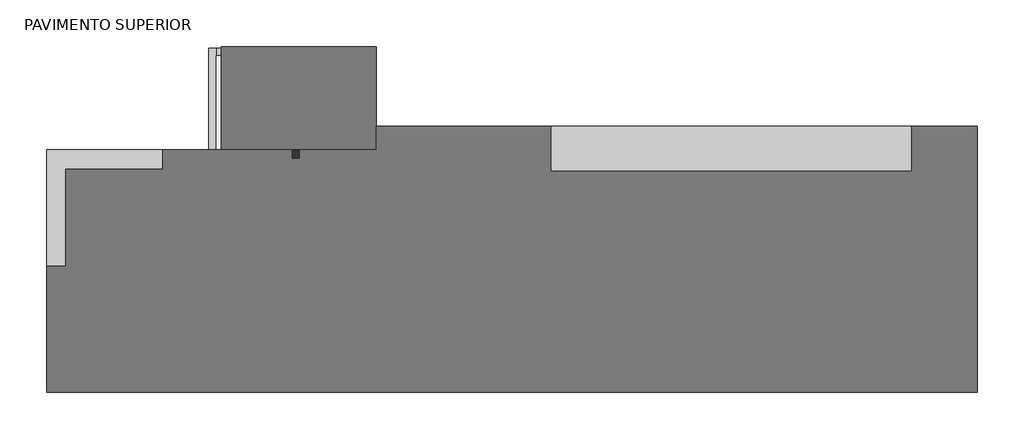
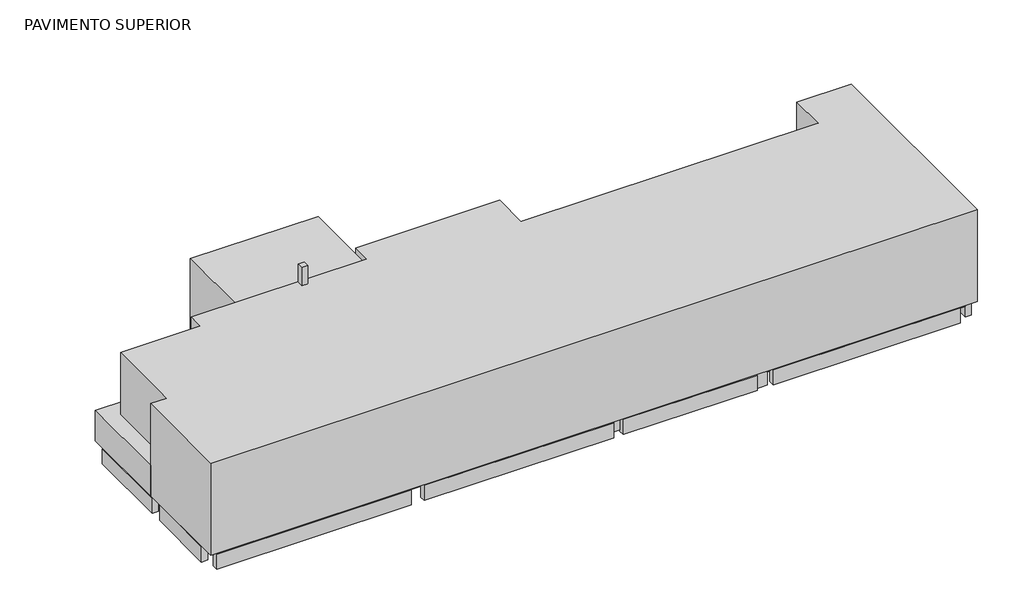
# One storey: 21 beams, 14 slabs, 2 proxies, 1 column.
"""IFC4 building model written with IfcOpenShell, lengths in millimetres."""

from ifc_helpers import new_model, si_unit, frame, origin, place, context, project, spatial, polyline, outline, extrude, faceted_brep, element, save

model = new_model("IFC4")

# Units and contexts
model_context = context("Model", 3, world=origin())
ifc_project = project(units=[si_unit("LENGTHUNIT", "METRE", prefix="MILLI")], contexts=[model_context])

# Site, building, storey
site = spatial("IfcSite", under=ifc_project)
building = spatial("IfcBuilding", under=site)
storey = spatial("IfcBuildingStorey", under=building, Name="PAVIMENTO SUPERIOR", Elevation=3600.0)

# Beams
placement = place(None, origin())
element("IfcBeam", 1, ObjectType="TQS - Viga retangular : 14.0 x 30.0", at=placement, inside=storey, context=model_context, shape_type="Brep", body=[
    faceted_brep([(10797.718693, -7454.5699847, 3530.0), (10797.718693, -7314.5699847, 3530.0), (9538.318693, -7314.5699847, 3530.0), (9538.318693, -7454.5699847, 3530.0), (10797.718693, -7454.5699847, 3230.0), (10797.718693, -7454.5699847, 3380.0), (9538.318693, -7454.5699847, 3380.0), (9538.318693, -7454.5699847, 3230.0), (10797.718693, -7314.5699847, 3230.0), (9538.318693, -7314.5699847, 3230.0), (10797.718693, -7314.5699847, 3380.0), (9538.318693, -7314.5699847, 3380.0)], [[[0, 1, 2, 3]], [[4, 5, 0, 3, 6, 7]], [[8, 4, 7, 9]], [[1, 10, 8, 9, 11, 2]], [[1, 0, 5, 4, 8, 10]], [[3, 2, 11, 9, 7, 6]]]),
])
element("IfcBeam", 2, ObjectType="TQS - Viga retangular : 14.0 x 50.0", at=placement, inside=storey, context=model_context, shape_type="Brep", body=[
    faceted_brep([(-5442.731307, -10953.5699847, 3530.0), (-5302.731307, -10953.5699847, 3530.0), (-5302.731307, -6553.3699847, 3530.0), (-5442.731307, -6553.3699847, 3530.0), (-5302.731307, -10953.5699847, 3380.0), (-5302.731307, -10953.5699847, 3030.0), (-5302.731307, -6553.3699847, 3030.0), (-5302.731307, -6553.3699847, 3380.0), (-5442.731307, -10953.5699847, 3030.0), (-5442.731307, -6553.3699847, 3030.0), (-5442.731307, -10953.5699847, 3380.0), (-5442.731307, -6553.3699847, 3380.0)], [[[0, 1, 2, 3]], [[1, 4, 5, 6, 7, 2]], [[5, 8, 9, 6]], [[8, 10, 0, 3, 11, 9]], [[1, 0, 10, 8, 5, 4]], [[3, 2, 7, 6, 9, 11]]]),
])
element("IfcBeam", 3, ObjectType="TQS - Viga retangular : 14.0 x 50.0", at=placement, inside=storey, context=model_context, shape_type="Brep", body=[
    faceted_brep([(-4442.481307, -4565.5699847, 3530.0), (-4442.481307, -4425.5699847, 3530.0), (-4512.281307, -4425.5699847, 3530.0), (-4702.281307, -4425.5699847, 3530.0), (-6440.281307, -4425.5699847, 3530.0), (-6440.281307, -4565.5699847, 3530.0), (-4702.281307, -4565.5699847, 3530.0), (-4512.281307, -4565.5699847, 3530.0), (-4442.481307, -4565.5699847, 3030.0), (-6440.281307, -4565.5699847, 3030.0), (-4702.281307, -4565.5699847, 3030.0), (-4512.281307, -4565.5699847, 3030.0), (-4442.481307, -4425.5699847, 3030.0), (-6440.281307, -4425.5699847, 3030.0), (-4702.281307, -4425.5699847, 3030.0), (-4512.281307, -4425.5699847, 3030.0), (-6440.281307, -4425.5699847, 3380.0)], [[[0, 1, 2, 3, 4, 5, 6, 7]], [[8, 0, 7, 6, 5, 9, 10, 11]], [[12, 8, 11, 10, 9, 13, 14, 15]], [[1, 12, 15, 14, 13, 16, 4, 3, 2]], [[1, 0, 8, 12]], [[5, 4, 16, 13, 9]]]),
])
element("IfcBeam", 4, ObjectType="TQS - Viga retangular : 14.0 x 50.0", at=placement, inside=storey, context=model_context, shape_type="Brep", body=[
    faceted_brep([(-4478.0679558, -6553.3699847, 3030.0), (-4478.0679558, -6413.3699847, 3030.0), (-4478.0679558, -6413.3699847, 3530.0), (-4478.0679558, -6450.0457433, 3530.0), (-4478.0679558, -6553.3699847, 3530.0), (-4478.0679558, -6553.3699847, 3380.0), (-6440.281307, -6413.3699847, 3530.0), (-6440.281307, -6553.3699847, 3530.0), (-5442.731307, -6553.3699847, 3530.0), (-5302.731307, -6553.3699847, 3530.0), (-4512.281307, -6413.3699847, 3530.0), (-4702.281307, -6413.3699847, 3530.0), (-6440.281307, -6553.3699847, 3030.0), (-5442.731307, -6553.3699847, 3030.0), (-5302.731307, -6553.3699847, 3030.0), (-6440.281307, -6413.3699847, 3030.0), (-4702.281307, -6413.3699847, 3030.0), (-4512.281307, -6413.3699847, 3030.0), (-6440.281307, -6413.3699847, 3380.0)], [[[0, 1, 2, 3, 4, 5]], [[6, 7, 8, 9, 4, 3, 2, 10, 11]], [[7, 12, 13, 14, 0, 5, 4, 9, 8]], [[1, 0, 14, 13, 12, 15, 16, 17]], [[2, 1, 17, 16, 15, 18, 6, 11, 10]], [[7, 6, 18, 15, 12]]]),
    faceted_brep([(-6840.281307, -6413.3699847, 3530.0), (-6840.281307, -6553.3699847, 3530.0), (-6840.281307, -6553.3699847, 3030.0), (-6840.281307, -6413.3699847, 3030.0), (-8589.281307, -6413.3699847, 3530.0), (-8589.281307, -6553.3699847, 3530.0), (-8589.281307, -6553.3699847, 3380.0), (-8589.281307, -6553.3699847, 3030.0), (-8589.281307, -6413.3699847, 3030.0), (-8589.281307, -6413.3699847, 3380.0)], [[[0, 1, 2, 3]], [[1, 0, 4, 5]], [[2, 1, 5, 6, 7]], [[3, 2, 7, 8]], [[0, 3, 8, 9, 4]], [[5, 4, 9, 8, 7, 6]]]),
    faceted_brep([(-8779.281307, -6413.3699847, 3530.0), (-8779.281307, -6553.3699847, 3530.0), (-8779.281307, -6553.3699847, 3380.0), (-8779.281307, -6553.3699847, 3030.0), (-8779.281307, -6413.3699847, 3030.0), (-8779.281307, -6413.3699847, 3380.0), (-12740.2813069, -6413.3699847, 3530.0), (-12740.2813069, -6553.3699847, 3530.0), (-12740.2813069, -6553.3699847, 3380.0), (-12740.2813069, -6553.3699847, 3030.0), (-12740.2813069, -6413.3699847, 3030.0), (-8780.281307, -6413.3699847, 3030.0), (-12740.2813069, -6413.3699847, 3380.0)], [[[0, 1, 2, 3, 4, 5]], [[1, 0, 6, 7]], [[3, 2, 1, 7, 8, 9]], [[4, 3, 9, 10, 11]], [[0, 5, 4, 11, 10, 12, 6]], [[7, 6, 12, 10, 9, 8]]]),
])
element("IfcBeam", 5, ObjectType="TQS - Viga retangular : 14.0 x 50.0", at=placement, inside=storey, context=model_context, shape_type="Brep", body=[
    faceted_brep([(-6580.281307, -2284.5699847, 3530.0), (-6440.281307, -2284.5699847, 3530.0), (-6440.281307, -2284.5699847, 3030.0), (-6580.281307, -2284.5699847, 3030.0), (-6580.281307, -2325.5699847, 3530.0), (-6580.281307, -2515.5699847, 3530.0), (-6580.281307, -4975.5699847, 3530.0), (-6440.281307, -4975.5699847, 3530.0), (-6440.281307, -4565.5699847, 3530.0), (-6440.281307, -4425.5699847, 3530.0), (-6440.281307, -2515.5699847, 3530.0), (-6440.281307, -2325.5699847, 3530.0), (-6440.281307, -4975.5699847, 3030.0), (-6440.281307, -4565.5699847, 3030.0), (-6440.281307, -4425.5699847, 3030.0), (-6440.281307, -2515.5699847, 3030.0), (-6440.281307, -2325.5699847, 3030.0), (-6580.281307, -4975.5699847, 3030.0), (-6580.281307, -2515.5699847, 3030.0), (-6580.281307, -2325.5699847, 3030.0)], [[[0, 1, 2, 3]], [[1, 0, 4, 5, 6, 7, 8, 9, 10, 11]], [[2, 1, 11, 10, 9, 8, 7, 12, 13, 14, 15, 16]], [[3, 2, 16, 15, 14, 13, 12, 17, 18, 19]], [[0, 3, 19, 18, 17, 6, 5, 4]], [[7, 6, 17, 12]]]),
    faceted_brep([(-6580.281307, -5165.5699847, 3530.0), (-6440.281307, -5165.5699847, 3530.0), (-6440.281307, -5165.5699847, 3030.0), (-6580.281307, -5165.5699847, 3030.0), (-6580.281307, -6413.3699847, 3530.0), (-6440.281307, -6413.3699847, 3530.0), (-6440.281307, -5594.3699847, 3530.0), (-6440.281307, -6413.3699847, 3380.0), (-6440.281307, -6413.3699847, 3030.0), (-6580.281307, -6413.3699847, 3030.0), (-6580.281307, -6413.3699847, 3380.0)], [[[0, 1, 2, 3]], [[1, 0, 4, 5, 6]], [[2, 1, 6, 5, 7, 8]], [[3, 2, 8, 9]], [[0, 3, 9, 10, 4]], [[5, 4, 10, 9, 8, 7]]]),
])
element("IfcBeam", 6, ObjectType="TQS - Viga retangular : 19.0 x 45.0", at=placement, inside=storey, context=model_context, shape_type="Brep", body=[
    faceted_brep([(-202.281307, -10953.5699847, 3530.0), (-12.281307, -10953.5699847, 3530.0), (-12.281307, -5715.5699847, 3530.0), (-12.281307, -5525.5699847, 3530.0), (-12.281307, -4775.5699847, 3530.0), (-202.281307, -4775.5699847, 3530.0), (-202.281307, -5546.7699847, 3530.0), (-202.281307, -6623.1699847, 3530.0), (-12.281307, -10953.5699847, 3380.0), (-12.281307, -10953.5699847, 3080.0), (-12.281307, -5715.5699847, 3080.0), (-12.281307, -5525.5699847, 3080.0), (-12.281307, -4775.5699847, 3080.0), (-202.281307, -10953.5699847, 3080.0), (-202.281307, -4775.5699847, 3080.0), (-202.281307, -10953.5699847, 3380.0)], [[[0, 1, 2, 3, 4, 5, 6, 7]], [[1, 8, 9, 10, 11, 12, 4, 3, 2]], [[9, 13, 14, 12, 11, 10]], [[13, 15, 0, 7, 6, 5, 14]], [[5, 4, 12, 14]], [[0, 15, 13, 9, 8, 1]]]),
])
element("IfcBeam", 7, ObjectType="TQS - Viga retangular : 19.0 x 45.0", at=placement, inside=storey, context=model_context, shape_type="Brep", body=[
    faceted_brep([(9348.318693, -10953.5699847, 3530.0), (9538.318693, -10953.5699847, 3530.0), (9538.318693, -7454.5699847, 3530.0), (9538.318693, -7314.5699847, 3530.0), (9538.318693, -4565.5699847, 3530.0), (9348.318693, -4565.5699847, 3530.0), (9348.318693, -5525.5699847, 3530.0), (9348.318693, -5715.5699847, 3530.0), (9538.318693, -10953.5699847, 3380.0), (9538.318693, -10953.5699847, 3080.0), (9538.318693, -4565.5699847, 3080.0), (9538.318693, -4565.5699847, 3380.0), (9348.318693, -10953.5699847, 3080.0), (9348.318693, -5715.5699847, 3080.0), (9348.318693, -5525.5699847, 3080.0), (9348.318693, -4565.5699847, 3080.0), (9348.318693, -10953.5699847, 3380.0), (9348.318693, -4565.5699847, 3440.0), (9348.318693, -4565.5699847, 3290.0)], [[[0, 1, 2, 3, 4, 5, 6, 7]], [[1, 8, 9, 10, 11, 4, 3, 2]], [[9, 12, 13, 14, 15, 10]], [[12, 16, 0, 7, 6, 5, 17, 18, 15, 14, 13]], [[1, 0, 16, 12, 9, 8]], [[5, 4, 11, 10, 15, 18, 17]]]),
])
element("IfcBeam", 8, ObjectType="TQS - Viga retangular : 19.0 x 45.0", at=placement, inside=storey, context=model_context, shape_type="Brep", body=[
    faceted_brep([(-12.281307, -5525.5699847, 3530.0), (-12.281307, -5715.5699847, 3530.0), (4253.718693, -5715.5699847, 3530.0), (4603.718693, -5715.5699847, 3530.0), (9348.318693, -5715.5699847, 3530.0), (9348.318693, -5525.5699847, 3530.0), (-12.281307, -5715.5699847, 3380.0), (-12.281307, -5715.5699847, 3080.0), (4253.718693, -5715.5699847, 3080.0), (4603.718693, -5715.5699847, 3080.0), (9348.318693, -5715.5699847, 3080.0), (9348.318693, -5715.5699847, 3380.0), (-12.281307, -5525.5699847, 3080.0), (4253.718693, -5525.5699847, 3080.0), (4603.718693, -5525.5699847, 3080.0), (9348.318693, -5525.5699847, 3080.0), (-12.281307, -5525.5699847, 3290.0), (-12.281307, -5525.5699847, 3440.0), (9348.318693, -5525.5699847, 3440.0), (9348.318693, -5525.5699847, 3290.0)], [[[0, 1, 2, 3, 4, 5]], [[1, 6, 7, 8, 9, 10, 11, 4, 3, 2]], [[7, 12, 13, 14, 15, 10, 9, 8]], [[12, 16, 17, 0, 5, 18, 19, 15, 14, 13]], [[1, 0, 17, 16, 12, 7, 6]], [[5, 4, 11, 10, 15, 19, 18]]]),
])
element("IfcBeam", 9, ObjectType="TQS - Viga retangular : 19.0 x 50.0", at=placement, inside=storey, context=model_context, shape_type="Brep", body=[
    faceted_brep([(-6649.181307, -11143.5699847, 3530.0), (-6649.181307, -10953.5699847, 3530.0), (-12740.2813069, -10953.5699847, 3530.0), (-12740.2813069, -11143.5699847, 3530.0), (-6649.181307, -11143.5699847, 3030.0), (-12740.2813069, -11143.5699847, 3030.0), (-6649.181307, -10953.5699847, 3030.0), (-12740.2813069, -10953.5699847, 3030.0), (-12740.2813069, -10953.5699847, 3380.0)], [[[0, 1, 2, 3]], [[4, 0, 3, 5]], [[6, 4, 5, 7]], [[1, 6, 7, 8, 2]], [[1, 0, 4, 6]], [[2, 8, 7, 5, 3]]]),
])
element("IfcBeam", 10, ObjectType="TQS - Viga retangular : 19.0 x 50.0", at=placement, inside=storey, context=model_context, shape_type="Brep", body=[
    faceted_brep([(-312.281307, -11143.5699847, 3530.0), (-312.281307, -10953.5699847, 3530.0), (-5302.731307, -10953.5699847, 3530.0), (-5442.731307, -10953.5699847, 3530.0), (-6249.181307, -10953.5699847, 3530.0), (-6249.181307, -11143.5699847, 3530.0), (-312.281307, -11143.5699847, 3030.0), (-6249.181307, -11143.5699847, 3030.0), (-312.281307, -10953.5699847, 3030.0), (-6249.181307, -10953.5699847, 3030.0), (-5442.731307, -10953.5699847, 3030.0), (-5302.731307, -10953.5699847, 3030.0)], [[[0, 1, 2, 3, 4, 5]], [[6, 0, 5, 7]], [[8, 6, 7, 9, 10, 11]], [[1, 8, 11, 10, 9, 4, 3, 2]], [[1, 0, 6, 8]], [[4, 9, 7, 5]]]),
])
element("IfcBeam", 11, ObjectType="TQS - Viga retangular : 19.0 x 50.0", at=placement, inside=storey, context=model_context, shape_type="Brep", body=[
    faceted_brep([(-12.281307, -10953.5699847, 3530.0), (-12.281307, -11143.5699847, 3530.0), (4178.718693, -11143.5699847, 3530.0), (4178.718693, -10953.5699847, 3530.0), (-12.281307, -11143.5699847, 3030.0), (4178.718693, -11143.5699847, 3030.0), (-12.281307, -10953.5699847, 3030.0), (4178.718693, -10953.5699847, 3030.0), (-12.281307, -10953.5699847, 3380.0)], [[[0, 1, 2, 3]], [[1, 4, 5, 2]], [[4, 6, 7, 5]], [[6, 8, 0, 3, 7]], [[3, 2, 5, 7]], [[0, 8, 6, 4, 1]]]),
    faceted_brep([(4678.718693, -11143.5699847, 3530.0), (4678.718693, -10953.5699847, 3530.0), (4678.718693, -10953.5699847, 3030.0), (4678.718693, -11143.5699847, 3030.0), (10537.718693, -11143.5699847, 3530.0), (10537.718693, -10953.5699847, 3530.0), (9538.318693, -10953.5699847, 3530.0), (9348.318693, -10953.5699847, 3530.0), (10537.718693, -11143.5699847, 3030.0), (10537.718693, -10953.5699847, 3030.0)], [[[0, 1, 2, 3]], [[4, 5, 6, 7, 1, 0]], [[8, 4, 0, 3]], [[9, 8, 3, 2]], [[5, 9, 2, 1, 7, 6]], [[5, 4, 8, 9]]]),
])
element("IfcBeam", 12, ObjectType="TQS - Viga retangular : 19.0 x 50.0", at=placement, inside=storey, context=model_context, shape_type="Brep", body=[
    faceted_brep([(-12930.2813069, -10643.5699847, 3530.0), (-12740.2813069, -10643.5699847, 3530.0), (-12740.2813069, -8375.5699847, 3530.0), (-12930.2813069, -8375.5699847, 3530.0), (-12740.2813069, -10643.5699847, 3030.0), (-12740.2813069, -8375.5699847, 3030.0), (-12930.2813069, -10643.5699847, 3030.0), (-12930.2813069, -8375.5699847, 3030.0)], [[[0, 1, 2, 3]], [[1, 4, 5, 2]], [[4, 6, 7, 5]], [[6, 0, 3, 7]], [[3, 2, 5, 7]], [[0, 6, 4, 1]]]),
    faceted_brep([(-12740.2813069, -7975.5699847, 3530.0), (-12930.2813069, -7975.5699847, 3530.0), (-12930.2813069, -7975.5699847, 3030.0), (-12740.2813069, -7975.5699847, 3030.0), (-12740.2813069, -5275.5699847, 3530.0), (-12930.2813069, -5275.5699847, 3530.0), (-12740.2813069, -6553.3699847, 3530.0), (-12740.2813069, -6413.3699847, 3530.0), (-12740.2813069, -5275.5699847, 3030.0), (-12740.2813069, -6553.3699847, 3030.0), (-12740.2813069, -6413.3699847, 3030.0), (-12930.2813069, -5275.5699847, 3030.0)], [[[0, 1, 2, 3]], [[4, 5, 1, 0, 6, 7]], [[8, 4, 7, 6, 0, 3, 9, 10]], [[11, 8, 10, 9, 3, 2]], [[5, 11, 2, 1]], [[5, 4, 8, 11]]]),
])
element("IfcBeam", 13, ObjectType="TQS - Viga retangular : 19.0 x 50.0", at=placement, inside=storey, context=model_context, shape_type="Brep", body=[
    faceted_brep([(4678.718693, -4375.5699847, 3530.0), (4678.718693, -4565.5699847, 3530.0), (9348.318693, -4565.5699847, 3530.0), (9538.318693, -4565.5699847, 3530.0), (10637.718693, -4565.5699847, 3530.0), (10637.718693, -4375.5699847, 3530.0), (4678.718693, -4565.5699847, 3440.0), (4678.718693, -4565.5699847, 3290.0), (4678.718693, -4565.5699847, 3030.0), (10637.718693, -4565.5699847, 3030.0), (4678.718693, -4375.5699847, 3030.0), (10637.718693, -4375.5699847, 3030.0)], [[[0, 1, 2, 3, 4, 5]], [[1, 6, 7, 8, 9, 4, 3, 2]], [[8, 10, 11, 9]], [[10, 0, 5, 11]], [[1, 0, 10, 8, 7, 6]], [[5, 4, 9, 11]]]),
    faceted_brep([(4178.718693, -4375.5699847, 3530.0), (4178.718693, -4565.5699847, 3530.0), (4178.718693, -4565.5699847, 3440.0), (4178.718693, -4565.5699847, 3290.0), (4178.718693, -4565.5699847, 3030.0), (4178.718693, -4375.5699847, 3030.0), (-12.281307, -4375.5699847, 3530.0), (-12.281307, -4565.5699847, 3530.0), (-12.281307, -4565.5699847, 3440.0), (-12.281307, -4565.5699847, 3290.0), (-12.281307, -4565.5699847, 3030.0), (-12.281307, -4375.5699847, 3030.0)], [[[0, 1, 2, 3, 4, 5]], [[0, 6, 7, 1]], [[1, 7, 8, 9, 10, 4, 3, 2]], [[4, 10, 11, 5]], [[6, 0, 5, 11]], [[6, 11, 10, 9, 8, 7]]]),
])
element("IfcBeam", 14, ObjectType="TQS - Viga retangular : 19.0 x 50.0", at=placement, inside=storey, context=model_context, shape_type="Brep", body=[
    faceted_brep([(10797.718693, -10953.5699847, 3530.0), (10987.718693, -10953.5699847, 3530.0), (10987.718693, -4565.5699847, 3530.0), (10797.718693, -4565.5699847, 3530.0), (10797.718693, -7314.5699847, 3530.0), (10797.718693, -7454.5699847, 3530.0), (10987.718693, -10953.5699847, 3030.0), (10987.718693, -4565.5699847, 3030.0), (10797.718693, -10953.5699847, 3030.0), (10797.718693, -4565.5699847, 3030.0), (10797.718693, -10953.5699847, 3380.0), (10797.718693, -4565.5699847, 3380.0)], [[[0, 1, 2, 3, 4, 5]], [[1, 6, 7, 2]], [[6, 8, 9, 7]], [[8, 10, 0, 5, 4, 3, 11, 9]], [[3, 2, 7, 9, 11]], [[0, 10, 8, 6, 1]]]),
])
element("IfcBeam", 15, ObjectType="TQS - Viga retangular : 19.0 x 50.0", at=placement, inside=storey, context=model_context, shape_type="Brep", body=[
    faceted_brep([(-6818.9099601, -5165.5699847, 3530.0), (-6840.281307, -5165.5699847, 3530.0), (-6840.281307, -4977.3842688, 3530.0), (-8589.281307, -4976.8464412, 3530.0), (-8589.281307, -5166.8464502, 3530.0), (-6818.91052, -5167.3908495, 3530.0), (-8589.281307, -5166.8464502, 3030.0), (-6818.91052, -5167.3908495, 3030.0), (-6840.281307, -5165.5699847, 3030.0), (-6818.9099601, -5165.5699847, 3030.0), (-8589.281307, -4976.8464412, 3030.0), (-6840.281307, -4977.3842688, 3030.0), (-8589.281307, -4976.8464412, 3380.0), (-6840.281307, -4977.3842688, 3380.0)], [[[0, 1, 2, 3, 4, 5]], [[5, 4, 6, 7]], [[8, 9, 7, 6, 10, 11]], [[11, 10, 12, 3, 2, 13]], [[8, 1, 0, 9]], [[1, 8, 11, 13, 2]], [[4, 3, 12, 10, 6]], [[5, 7, 9, 0]]]),
    faceted_brep([(-8779.281307, -4976.7880151, 3530.0), (-8779.281307, -5166.7880241, 3530.0), (-8779.281307, -5166.7880241, 3380.0), (-8779.281307, -5166.7880241, 3030.0), (-8779.281307, -4976.7880151, 3030.0), (-12740.31052, -5165.5699847, 3530.0), (-12740.2520939, -4975.5699937, 3530.0), (-12740.31052, -5165.5699847, 3030.0), (-8780.281307, -5166.7877166, 3030.0), (-12740.2520939, -4975.5699937, 3030.0)], [[[0, 1, 2, 3, 4]], [[5, 1, 0, 6]], [[1, 5, 7, 8, 3, 2]], [[3, 8, 7, 9, 4]], [[4, 9, 6, 0]], [[6, 9, 7, 5]]]),
])
element("IfcBeam", 16, ObjectType="TQS - Viga retangular : 19.0 x 50.0", at=placement, inside=storey, context=model_context, shape_type="Brep", body=[
    faceted_brep([(-8779.281307, -4975.5699847, 3530.0), (-8590.281307, -4975.5699847, 3530.0), (-8590.281307, -2515.5699847, 3530.0), (-8590.281307, -2325.5699847, 3530.0), (-8780.281307, -2325.5699847, 3530.0), (-8780.281307, -4976.7877076, 3530.0), (-8779.281307, -4976.7880151, 3530.0), (-8590.281307, -4975.5699847, 3030.0), (-8590.281307, -2515.5699847, 3030.0), (-8590.281307, -2325.5699847, 3030.0), (-8779.281307, -4975.5699847, 3030.0), (-8779.281307, -4976.7880151, 3030.0), (-8780.281307, -4976.7877076, 3030.0), (-8780.281307, -2325.5699847, 3030.0)], [[[0, 1, 2, 3, 4, 5, 6]], [[1, 7, 8, 9, 3, 2]], [[7, 10, 11, 12, 13, 9, 8]], [[12, 5, 4, 13]], [[0, 10, 7, 1]], [[6, 5, 12, 11]], [[10, 0, 6, 11]], [[4, 3, 9, 13]]]),
    faceted_brep([(-8779.281307, -6413.3699847, 3030.0), (-8779.281307, -5166.7880241, 3030.0), (-8779.281307, -5166.7880241, 3380.0), (-8779.281307, -6413.3699847, 3380.0), (-8780.281307, -5166.7877166, 3030.0), (-8780.281307, -5166.7877166, 3380.0), (-8780.281307, -6413.3699847, 3030.0), (-8780.281307, -6413.3699847, 3380.0)], [[[0, 1, 2, 3]], [[1, 4, 5, 2]], [[4, 1, 0, 6]], [[4, 6, 7, 5]], [[6, 0, 3, 7]], [[3, 2, 5, 7]]]),
])
element("IfcBeam", 17, ObjectType="TQS - Viga retangular : 19.0 x 50.0", at=placement, inside=storey, context=model_context, shape_type="Brep", body=[
    faceted_brep([(-4702.281307, -4425.5699847, 3530.0), (-4512.281307, -4425.5699847, 3530.0), (-4512.281307, -2325.5699847, 3530.0), (-4702.281307, -2325.5699847, 3530.0), (-4702.281307, -2515.5699847, 3530.0), (-4512.281307, -4425.5699847, 3030.0), (-4512.281307, -2325.5699847, 3030.0), (-4702.281307, -4425.5699847, 3030.0), (-4702.281307, -2515.5699847, 3030.0), (-4702.281307, -2325.5699847, 3030.0), (-4702.281307, -4425.5699847, 3380.0)], [[[0, 1, 2, 3, 4]], [[1, 5, 6, 2]], [[5, 7, 8, 9, 6]], [[7, 10, 0, 4, 3, 9, 8]], [[1, 0, 10, 7, 5]], [[3, 2, 6, 9]]]),
    faceted_brep([(-4702.281307, -4565.5699847, 3530.0), (-4512.281307, -4565.5699847, 3530.0), (-4512.281307, -4565.5699847, 3030.0), (-4702.281307, -4565.5699847, 3030.0), (-4702.281307, -5594.3699847, 3530.0), (-4702.281307, -6413.3699847, 3530.0), (-4512.281307, -6413.3699847, 3530.0), (-4512.281307, -6413.3699847, 3030.0), (-4702.281307, -6413.3699847, 3030.0), (-4702.281307, -6413.3699847, 3380.0)], [[[0, 1, 2, 3]], [[1, 0, 4, 5, 6]], [[2, 1, 6, 7]], [[3, 2, 7, 8]], [[0, 3, 8, 9, 5, 4]], [[6, 5, 9, 8, 7]]]),
])
element("IfcBeam", 18, ObjectType="TQS - Viga retangular : 19.0 x 50.0", at=placement, inside=storey, context=model_context, shape_type="Brep", body=[
    faceted_brep([(-6440.281307, -2325.5699847, 3530.0), (-6440.281307, -2515.5699847, 3530.0), (-4702.281307, -2515.5699847, 3530.0), (-4702.281307, -2325.5699847, 3530.0), (-6440.281307, -2515.5699847, 3380.0), (-6440.281307, -2515.5699847, 3030.0), (-4702.281307, -2515.5699847, 3030.0), (-4702.281307, -2515.5699847, 3380.0), (-6440.281307, -2325.5699847, 3030.0), (-4702.281307, -2325.5699847, 3030.0)], [[[0, 1, 2, 3]], [[1, 4, 5, 6, 7, 2]], [[5, 8, 9, 6]], [[8, 0, 3, 9]], [[1, 0, 8, 5, 4]], [[3, 2, 7, 6, 9]]]),
    faceted_brep([(-6580.281307, -2325.5699847, 3530.0), (-6580.281307, -2515.5699847, 3530.0), (-6580.281307, -2515.5699847, 3380.0), (-6580.281307, -2515.5699847, 3030.0), (-6580.281307, -2325.5699847, 3030.0), (-8590.281307, -2325.5699847, 3530.0), (-8590.281307, -2515.5699847, 3530.0), (-8590.281307, -2515.5699847, 3030.0), (-8590.281307, -2325.5699847, 3030.0)], [[[0, 1, 2, 3, 4]], [[1, 0, 5, 6]], [[3, 2, 1, 6, 7]], [[4, 3, 7, 8]], [[0, 4, 8, 5]], [[6, 5, 8, 7]]]),
])
element("IfcBeam", 19, ObjectType="TQS - Viga retangular : 19.0 x 50.0", at=placement, inside=storey, context=model_context, shape_type="SweptSolid", body=[
    extrude(outline(polyline([(-202.281307, -4375.5699847), (-202.281307, -4565.5699847), (-4142.481307, -4565.5699847), (-4142.481307, -4375.5699847), (-202.281307, -4375.5699847)])), frame((0.0, 0.0, 3030.0), z_axis=(0.0, 0.0, 1.0), x_axis=(1.0, 0.0, 0.0)), (0.0, 0.0, 1.0), 500.0),
])
element("IfcBeam", 20, ObjectType="TQS - Viga retangular : 35.0 x 50.0", at=placement, inside=storey, context=model_context, shape_type="Brep", body=[
    faceted_brep([(4253.718693, -5525.5699847, 3440.0), (4253.718693, -5525.5699847, 3290.0), (4253.718693, -5525.5699847, 3080.0), (4253.718693, -5525.5699847, 2940.0), (4603.718693, -5525.5699847, 2940.0), (4603.718693, -5525.5699847, 3080.0), (4603.718693, -5525.5699847, 3290.0), (4603.718693, -5525.5699847, 3440.0), (4603.718693, -4584.5699847, 3440.0), (4253.718693, -4584.5699847, 3440.0), (4603.718693, -4584.5699847, 2940.0), (4603.718693, -4584.5699847, 3290.0), (4253.718693, -4584.5699847, 2940.0), (4253.718693, -4584.5699847, 3290.0)], [[[0, 1, 2, 3, 4, 5, 6, 7]], [[8, 9, 0, 7]], [[10, 11, 8, 7, 6, 5, 4]], [[12, 10, 4, 3]], [[9, 13, 12, 3, 2, 1, 0]], [[9, 8, 11, 10, 12, 13]]]),
])
element("IfcBeam", 21, ObjectType="TQS - Viga retangular : 35.0 x 59.0", at=placement, inside=storey, context=model_context, shape_type="Brep", body=[
    faceted_brep([(4253.718693, -10953.5699847, 3530.0), (4603.718693, -10953.5699847, 3530.0), (4603.718693, -5715.5699847, 3530.0), (4253.718693, -5715.5699847, 3530.0), (4603.718693, -10953.5699847, 3380.0), (4603.718693, -10953.5699847, 2940.0), (4603.718693, -5525.5699847, 2940.0), (4603.718693, -5525.5699847, 3080.0), (4603.718693, -5715.5699847, 3080.0), (4603.718693, -5715.5699847, 3380.0), (4253.718693, -10953.5699847, 2940.0), (4253.718693, -5525.5699847, 2940.0), (4253.718693, -10953.5699847, 3380.0), (4253.718693, -5715.5699847, 3380.0), (4253.718693, -5715.5699847, 3080.0), (4253.718693, -5525.5699847, 3080.0)], [[[0, 1, 2, 3]], [[1, 4, 5, 6, 7, 8, 9, 2]], [[5, 10, 11, 6]], [[10, 12, 0, 3, 13, 14, 15, 11]], [[0, 12, 10, 5, 4, 1]], [[6, 11, 15, 7]], [[8, 14, 13, 3, 2, 9]], [[14, 8, 7, 15]]]),
])

# Proxies
element("IfcBuildingElementProxy", 22, Name="SUÍTES E SALA ÍNTIMA : SUÍTES E SALA ÍNTIMA", ObjectType="SUÍTES E SALA ÍNTIMA : SUÍTES E SALA ÍNTIMA", at=placement, inside=storey, context=model_context, shape_type="SolidModel", body=[
    faceted_brep([(-12960.281307, -11195.5699847, 3600.0), (11039.718693, -11195.5699847, 3600.0), (11039.718693, -11195.5699847, 6650.0), (-12960.281307, -11195.5699847, 6650.0), (11039.718693, -4345.5699847, 3600.0), (11039.718693, -4345.5699847, 6650.0), (9339.718693, -4345.5699847, 3600.0), (9339.718693, -4345.5699847, 6650.0), (9339.718693, -5495.5699847, 3600.0), (9339.718693, -5495.5699847, 6650.0), (39.718693, -5495.5699847, 3600.0), (39.718693, -5495.5699847, 6650.0), (39.718693, -4345.5699847, 3600.0), (39.718693, -4345.5699847, 6650.0), (-4460.281307, -4345.5699847, 3600.0), (-4460.281307, -4345.5699847, 6650.0), (-4460.281307, -4595.5699847, 3600.0), (-4460.281307, -4595.5699847, 4700.0), (-4460.281307, -4945.5699847, 4700.0), (-4460.281307, -4945.5699847, 6650.0), (-9960.281307, -4945.5699847, 3600.0), (-9960.281307, -4945.5699847, 6650.0), (-6410.281307, -4945.5699847, 4700.0), (-6410.281307, -4945.5699847, 3600.0), (-9960.281307, -5445.5699847, 3600.0), (-9960.281307, -5445.5699847, 6650.0), (-12460.281307, -5445.5699847, 3600.0), (-12460.281307, -5445.5699847, 6650.0), (-12460.281307, -7945.5699847, 3600.0), (-12460.281307, -7945.5699847, 6650.0), (-12960.281307, -7945.5699847, 3600.0), (-12960.281307, -7945.5699847, 6650.0), (-6410.281307, -5595.5699847, 3600.0), (-4457.4976512, -5595.5699847, 3600.0), (-4457.4976512, -4595.5699847, 3600.0), (-210.281307, -4595.5699847, 3600.0), (-1217.4976512, -4595.5699847, 3600.0), (-1217.4976512, -5515.5699847, 3600.0), (-210.281307, -5515.5699847, 3600.0), (-210.281307, -4595.5699847, 4700.0), (-1217.4976512, -4595.5699847, 4700.0), (-1217.4976512, -5515.5699847, 4700.0), (-210.281307, -5515.5699847, 4700.0), (-4457.4976512, -4595.5699847, 4700.0), (-6410.281307, -5595.5699847, 4700.0), (-4457.4976512, -5595.5699847, 4700.0)], [[[0, 1, 2, 3]], [[2, 1, 4, 5]], [[5, 4, 6, 7]], [[7, 6, 8, 9]], [[9, 8, 10, 11]], [[11, 10, 12, 13]], [[13, 12, 14, 15]], [[15, 14, 16, 17, 18, 19]], [[20, 21, 19, 18, 22, 23]], [[21, 20, 24, 25]], [[25, 24, 26, 27]], [[27, 26, 28, 29]], [[29, 28, 30, 31]], [[0, 3, 31, 30]], [[3, 2, 5, 7, 9, 11, 13, 15, 19, 21, 25, 27, 29, 31]], [[1, 0, 30, 28, 26, 24, 20, 23, 32, 33, 34, 16, 14, 12, 10, 8, 6, 4], [35, 36, 37, 38]], [[35, 39, 40, 36]], [[36, 40, 41, 37]], [[37, 41, 42, 38]], [[39, 35, 38, 42]], [[40, 39, 42, 41]], [[34, 43, 17, 16]], [[44, 32, 23, 22]], [[32, 44, 45, 33]], [[43, 34, 33, 45]], [[45, 44, 22, 18, 17, 43]]]),
    faceted_brep([(-4460.281307, -2295.5699847, 3600.0), (-8460.281307, -2295.5699847, 3600.0), (-8460.281307, -2295.5699847, 6450.0), (-4460.281307, -2295.5699847, 6450.0), (-8460.281307, -4945.5699847, 3600.0), (-8460.281307, -4945.5699847, 6450.0), (-6410.281307, -4945.5699847, 3600.0), (-6410.281307, -4945.5699847, 4700.0), (-4460.281307, -4945.5699847, 4700.0), (-4460.281307, -4945.5699847, 6450.0), (-4460.281307, -4595.5699847, 4700.0), (-4460.281307, -4595.5699847, 3600.0), (-6410.281307, -4595.5699847, 3600.0), (-6410.281307, -4595.5699847, 4700.0)], [[[0, 1, 2, 3]], [[2, 1, 4, 5]], [[5, 4, 6, 7, 8, 9]], [[0, 3, 9, 8, 10, 11]], [[3, 2, 5, 9]], [[1, 0, 11, 12, 6, 4]], [[13, 12, 11, 10]], [[12, 13, 7, 6]], [[13, 10, 8, 7]]]),
    extrude(outline(polyline([(-9960.281307, -5445.5699847), (-12460.281307, -5445.5699847), (-12460.281307, -7945.5699847), (-12960.281307, -7945.5699847), (-12960.281307, -4945.5699847), (-9960.281307, -4945.5699847), (-9960.281307, -5445.5699847)])), frame((0.0, 0.0, 3600.0), z_axis=(0.0, 0.0, 1.0), x_axis=(1.0, 0.0, 0.0)), (0.0, 0.0, 1.0), 1000.0),
])
element("IfcBuildingElementProxy", 23, Name="TERRAÇO : TERRAÇO", ObjectType="TERRAÇO : TERRAÇO", at=placement, inside=storey, context=model_context, shape_type="SweptSolid", body=[
    extrude(outline(polyline([(39.718693, -4345.5699847), (9339.718693, -4345.5699847), (9339.718693, -5495.5699847), (39.718693, -5495.5699847), (39.718693, -4345.5699847)])), frame((0.0, 0.0, 3600.0), z_axis=(0.0, 0.0, 1.0), x_axis=(1.0, 0.0, 0.0)), (0.0, 0.0, 1.0), 1100.0),
])

# Column
element("IfcColumn", 24, ObjectType="TQS - Pilar retangular : 19.0 x 19.0", at=placement, inside=storey, context=model_context, shape_type="Brep", body=[
    faceted_brep([(-6630.281307, -5165.5699847, 3530.0), (-6630.281307, -4975.5699847, 3530.0), (-6440.281307, -4975.5699847, 3530.0), (-6440.281307, -5165.5699847, 3530.0), (-6630.281307, -5165.5699847, 7250.0), (-6630.281307, -4975.5699847, 7250.0), (-6630.281307, -4975.5699847, 6290.0), (-6630.281307, -5165.5699847, 6290.0), (-6440.281307, -4975.5699847, 7250.0), (-6440.281307, -4975.5699847, 7050.0), (-6440.281307, -4975.5699847, 6290.0), (-6440.281307, -5165.5699847, 7250.0), (-6440.281307, -5165.5699847, 7050.0), (-6440.281307, -5165.5699847, 6290.0)], [[[0, 1, 2, 3]], [[4, 5, 6, 1, 0, 7]], [[5, 8, 9, 10, 2, 1, 6]], [[8, 11, 12, 13, 3, 2, 10, 9]], [[11, 4, 7, 0, 3, 13, 12]], [[4, 11, 8, 5]]]),
])

# Slabs
element("IfcSlab", 25, ObjectType="TQS h=15", at=placement, inside=storey, context=model_context, shape_type="SweptSolid", body=[
    extrude(outline(polyline([(-4702.281307, -4425.5699847), (-6440.281307, -4425.5699847), (-6440.281307, -2515.5699847), (-4702.281307, -2515.5699847), (-4702.281307, -4425.5699847)])), frame((0.0, 0.0, 3380.0), z_axis=(0.0, 0.0, 1.0), x_axis=(1.0, 0.0, 0.0)), (0.0, 0.0, 1.0), 150.0),
])
element("IfcSlab", 26, ObjectType="TQS h=15", at=placement, inside=storey, context=model_context, shape_type="Brep", body=[
    faceted_brep([(-202.281307, -10953.5699847, 3380.0), (-5302.731307, -10953.5699847, 3380.0), (-5302.731307, -6553.3699847, 3380.0), (-4478.0679558, -6553.3699847, 3380.0), (-4478.0679558, -6450.0457433, 3380.0), (-4471.281307, -6450.0457433, 3380.0), (-4471.281307, -6623.1699847, 3380.0), (-202.281307, -6623.1699847, 3380.0), (-202.281307, -10953.5699847, 3530.0), (-202.281307, -6623.1699847, 3530.0), (-4471.281307, -6623.1699847, 3530.0), (-4471.281307, -6450.0457433, 3530.0), (-4478.0679558, -6450.0457433, 3530.0), (-4478.0679558, -6553.3699847, 3530.0), (-5302.731307, -6553.3699847, 3530.0), (-5302.731307, -10953.5699847, 3530.0), (-312.281307, -10953.5699847, 3530.0)], [[[0, 1, 2, 3, 4, 5, 6, 7]], [[8, 9, 10, 11, 12, 13, 14, 15, 16]], [[1, 0, 8, 16, 15]], [[2, 1, 15, 14]], [[3, 2, 14, 13]], [[4, 3, 13, 12]], [[5, 4, 12, 11]], [[6, 5, 11, 10]], [[7, 6, 10, 9]], [[0, 7, 9, 8]]]),
])
element("IfcSlab", 27, ObjectType="TQS h=15", at=placement, inside=storey, context=model_context, shape_type="Brep", body=[
    faceted_brep([(9348.318693, -5715.5699847, 3380.0), (9348.318693, -10953.5699847, 3380.0), (4603.718693, -10953.5699847, 3380.0), (4603.718693, -5715.5699847, 3380.0), (9348.318693, -5715.5699847, 3530.0), (4603.718693, -5715.5699847, 3530.0), (4603.718693, -10953.5699847, 3530.0), (4678.718693, -10953.5699847, 3530.0), (9348.318693, -10953.5699847, 3530.0)], [[[0, 1, 2, 3]], [[4, 5, 6, 7, 8]], [[1, 0, 4, 8]], [[2, 1, 8, 7, 6]], [[3, 2, 6, 5]], [[0, 3, 5, 4]]]),
])
element("IfcSlab", 28, ObjectType="TQS h=15", at=placement, inside=storey, context=model_context, shape_type="Brep", body=[
    faceted_brep([(-5442.731307, -10953.5699847, 3380.0), (-12740.2813069, -10953.5699847, 3380.0), (-12740.2813069, -6553.3699847, 3380.0), (-8779.281307, -6553.3699847, 3380.0), (-8589.281307, -6553.3699847, 3380.0), (-5442.731307, -6553.3699847, 3380.0), (-5442.731307, -10953.5699847, 3530.0), (-5442.731307, -6553.3699847, 3530.0), (-6440.281307, -6553.3699847, 3530.0), (-6840.281307, -6553.3699847, 3530.0), (-8589.281307, -6553.3699847, 3530.0), (-8779.281307, -6553.3699847, 3530.0), (-12740.2813069, -6553.3699847, 3530.0), (-12740.2813069, -7975.5699847, 3530.0), (-12740.2813069, -8375.5699847, 3530.0), (-12740.2813069, -10643.5699847, 3530.0), (-12740.2813069, -10953.5699847, 3530.0), (-6649.181307, -10953.5699847, 3530.0), (-6249.181307, -10953.5699847, 3530.0)], [[[0, 1, 2, 3, 4, 5]], [[6, 7, 8, 9, 10, 11, 12, 13, 14, 15, 16, 17, 18]], [[1, 0, 6, 18, 17, 16]], [[2, 1, 16, 15, 14, 13, 12]], [[5, 4, 3, 2, 12, 11, 10, 9, 8, 7]], [[0, 5, 7, 6]]]),
])
element("IfcSlab", 29, ObjectType="TQS h=15", at=placement, inside=storey, context=model_context, shape_type="Brep", body=[
    faceted_brep([(-8779.281307, -6413.3699847, 3380.0), (-8780.281307, -6413.3699847, 3380.0), (-12740.2813069, -6413.3699847, 3380.0), (-12740.2813069, -5165.5699937, 3380.0), (-8780.281307, -5166.7877166, 3380.0), (-8779.281307, -5166.7880241, 3380.0), (-8779.281307, -6413.3699847, 3530.0), (-8779.281307, -5166.7880241, 3530.0), (-12740.2813069, -5165.5699937, 3530.0), (-12740.2813069, -5275.5699847, 3530.0), (-12740.2813069, -6413.3699847, 3530.0)], [[[0, 1, 2, 3, 4, 5]], [[6, 7, 8, 9, 10]], [[2, 1, 0, 6, 10]], [[3, 2, 10, 9, 8]], [[5, 4, 3, 8, 7]], [[0, 5, 7, 6]]]),
])
element("IfcSlab", 30, ObjectType="TQS h=15", at=placement, inside=storey, context=model_context, shape_type="Brep", body=[
    faceted_brep([(-8589.281307, -5166.8464502, 3380.0), (-6840.281307, -5167.3842778, 3380.0), (-6580.281307, -5165.5699847, 3380.0), (-6580.281307, -6413.3699847, 3380.0), (-8589.281307, -6413.3699847, 3380.0), (-8589.281307, -5166.8464502, 3530.0), (-8589.281307, -6413.3699847, 3530.0), (-6840.281307, -6413.3699847, 3530.0), (-6580.281307, -6413.3699847, 3530.0), (-6580.281307, -5165.5699847, 3530.0), (-6840.281307, -5167.3842778, 3530.0)], [[[0, 1, 2, 3, 4]], [[5, 6, 7, 8, 9, 10]], [[1, 0, 5, 10]], [[2, 1, 10, 9]], [[3, 2, 9, 8]], [[4, 3, 8, 7, 6]], [[0, 4, 6, 5]]]),
])
element("IfcSlab", 31, ObjectType="TQS h=15", at=placement, inside=storey, context=model_context, shape_type="SweptSolid", body=[
    extrude(outline(polyline([(-6840.281307, -4977.3842688), (-8589.281307, -4976.8464412), (-8590.281307, -2515.5699847), (-6580.281307, -2515.5699847), (-6580.281307, -4975.5699847), (-6840.281307, -4977.3842688)])), frame((0.0, 0.0, 3380.0), z_axis=(0.0, 0.0, 1.0), x_axis=(1.0, 0.0, 0.0)), (0.0, 0.0, 1.0), 150.0),
])
element("IfcSlab", 32, ObjectType="TQS h=15", at=placement, inside=storey, context=model_context, shape_type="SweptSolid", body=[
    extrude(outline(polyline([(-4702.281307, -6413.3699847), (-6440.281307, -6413.3699847), (-6440.281307, -5594.3699847), (-4702.281307, -5594.3699847), (-4702.281307, -6413.3699847)])), frame((0.0, 0.0, 3380.0), z_axis=(0.0, 0.0, 1.0), x_axis=(1.0, 0.0, 0.0)), (0.0, 0.0, 1.0), 150.0),
])
element("IfcSlab", 33, ObjectType="TQS h=15", at=placement, inside=storey, context=model_context, shape_type="SweptSolid", body=[
    extrude(outline(polyline([(-1231.281307, -5546.7699847), (-202.281307, -5546.7699847), (-202.281307, -6623.1699847), (-1231.281307, -6623.1699847), (-1231.281307, -5546.7699847)])), frame((0.0, 0.0, 3380.0), z_axis=(0.0, 0.0, 1.0), x_axis=(1.0, 0.0, 0.0)), (0.0, 0.0, 1.0), 150.0),
])
element("IfcSlab", 34, ObjectType="TQS h=15", at=placement, inside=storey, context=model_context, shape_type="Brep", body=[
    faceted_brep([(4253.718693, -10953.5699847, 3380.0), (-12.281307, -10953.5699847, 3380.0), (-12.281307, -5715.5699847, 3380.0), (4253.718693, -5715.5699847, 3380.0), (4253.718693, -10953.5699847, 3530.0), (4253.718693, -5715.5699847, 3530.0), (-12.281307, -5715.5699847, 3530.0), (-12.281307, -10953.5699847, 3530.0), (4178.718693, -10953.5699847, 3530.0)], [[[0, 1, 2, 3]], [[4, 5, 6, 7, 8]], [[1, 0, 4, 8, 7]], [[2, 1, 7, 6]], [[3, 2, 6, 5]], [[0, 3, 5, 4]]]),
])
element("IfcSlab", 35, ObjectType="TQS h=15", at=placement, inside=storey, context=model_context, shape_type="Brep", body=[
    faceted_brep([(9538.318693, -7314.5699847, 3380.0), (9538.318693, -4565.5699847, 3380.0), (10797.718693, -4565.5699847, 3380.0), (10797.718693, -7314.5699847, 3380.0), (9538.318693, -7314.5699847, 3530.0), (10797.718693, -7314.5699847, 3530.0), (10797.718693, -4565.5699847, 3530.0), (10637.718693, -4565.5699847, 3530.0), (9538.318693, -4565.5699847, 3530.0)], [[[0, 1, 2, 3]], [[4, 5, 6, 7, 8]], [[1, 0, 4, 8]], [[2, 1, 8, 7, 6]], [[3, 2, 6, 5]], [[0, 3, 5, 4]]]),
])
element("IfcSlab", 36, ObjectType="TQS h=15", at=placement, inside=storey, context=model_context, shape_type="Brep", body=[
    faceted_brep([(10797.718693, -10953.5699847, 3380.0), (9538.318693, -10953.5699847, 3380.0), (9538.318693, -7454.5699847, 3380.0), (10797.718693, -7454.5699847, 3380.0), (10797.718693, -10953.5699847, 3530.0), (10797.718693, -7454.5699847, 3530.0), (9538.318693, -7454.5699847, 3530.0), (9538.318693, -10953.5699847, 3530.0), (10537.718693, -10953.5699847, 3530.0)], [[[0, 1, 2, 3]], [[4, 5, 6, 7, 8]], [[1, 0, 4, 8, 7]], [[2, 1, 7, 6]], [[3, 2, 6, 5]], [[0, 3, 5, 4]]]),
])
element("IfcSlab", 37, ObjectType="TQS h=15", at=placement, inside=storey, context=model_context, shape_type="SweptSolid", body=[
    extrude(outline(polyline([(-12.281307, -4565.5699847), (4178.718693, -4565.5699847), (4178.718693, -4584.5699847), (4253.718693, -4584.5699847), (4253.718693, -5525.5699847), (-12.281307, -5525.5699847), (-12.281307, -4565.5699847)])), frame((0.0, 0.0, 3290.0), z_axis=(0.0, 0.0, 1.0), x_axis=(1.0, 0.0, 0.0)), (0.0, 0.0, 1.0), 150.0),
])
element("IfcSlab", 38, ObjectType="TQS h=15", at=placement, inside=storey, context=model_context, shape_type="SweptSolid", body=[
    extrude(outline(polyline([(4678.718693, -4565.5699847), (9348.318693, -4565.5699847), (9348.318693, -5525.5699847), (4603.718693, -5525.5699847), (4603.718693, -4584.5699847), (4678.718693, -4584.5699847), (4678.718693, -4565.5699847)])), frame((0.0, 0.0, 3290.0), z_axis=(0.0, 0.0, 1.0), x_axis=(1.0, 0.0, 0.0)), (0.0, 0.0, 1.0), 150.0),
])

save(model, "model.ifc")

# Revit data of these elements
# Type "TQS - Viga retangular : 14.0 x 30.0"
#   Length [instance default] = 1.524 m
#   b = 0.14 m
#   h = 0.30 m
#   Structural Material [instance default] = none
#   Assembly Code = ""
# Type "TQS - Viga retangular : 14.0 x 50.0"
#   Length [instance default] = 1.524 m
#   b = 0.14 m
#   h = 0.50 m
#   Structural Material [instance default] = none
#   Assembly Code = ""
# Type "TQS - Viga retangular : 19.0 x 45.0"
#   Length [instance default] = 1.524 m
#   b = 0.19 m
#   h = 0.45 m
#   Structural Material [instance default] = none
#   Assembly Code = ""
# Type "TQS - Viga retangular : 19.0 x 50.0"
#   Length [instance default] = 1.524 m
#   b = 0.19 m
#   h = 0.50 m
#   Structural Material [instance default] = none
#   Assembly Code = ""
# Type "TQS - Viga retangular : 35.0 x 50.0"
#   Length [instance default] = 1.524 m
#   b = 0.35 m
#   h = 0.50 m
#   Structural Material [instance default] = none
#   Assembly Code = ""
# Type "TQS - Viga retangular : 35.0 x 59.0"
#   Length [instance default] = 1.524 m
#   b = 0.35 m
#   h = 0.59 m
#   Structural Material [instance default] = none
#   Assembly Code = ""
# Type "TQS - Pilar retangular : 19.0 x 19.0"
#   b = 0.19 m
#   h = 0.19 m
#   Structural Material [instance default] = Concrete - Cast-in-Place Concrete
# Type "TQS h=15"
#   Function = 0
#   Layers, outside or top first: 0.15 m ".MATERIAL GENÉRICO LAJE E PISO" (function 1)
# Element 1 (IfcBeam, "TQS - Viga retangular : 14.0 x 30.0")
#   Uso = "ESTRUTURA"
#   Titulo = "V208"
#   Chave = "-1334"
#   Tipo Elemento = "Viga"
#   SHA1 = "E6514DD7580E8C0F3F88343C2DB6E333F007C4CA"
#   Revisão = ""
#   Tipo de carga = ""
#   Divisor de flexao = ""
#   Secao = ""
#   Configuracao = ""
#   Angulo (graus) = ""
#   Detalhamento = ""
#   Casos de vento manual = ""
#   Tipo = ""
#   Alcas = ""
#   Furos = ""
#   Pino = ""
#   Distribuicao = ""
#   Solidarizado = ""
#   Solidarizar na montagem = ""
#   Unir com o próximo = ""
#   Grupo pre moldado = ""
#   Verificado = ""
#   Concreto C = ""
#   Taxa de armadura (kgf/m³) = 0
#   Carga (tf/m²) = 0
#   Carga (tf/m) = 0
#   Carga (tf) = 0
#   Altura = 0.30 m
#   Rebaixo = 0.07 m
#   Largura = 0.14 m
#   Distancia a face = 0.00 m
#   Distancia ao eixo = 0.00 m
#   Altura gerber esquerda = 0.00 m
#   Largura gerber esquerda = 0.00 m
#   Altura gerber direita = 0.00 m
#   Largura gerber direita = 0.00 m
#   Resultado de Ensaios fck (MPa) = 0
#   Unique TQS ID = -1334
#   Principal = yes
#   Structural Material = none
#   Phase Created = CC_AP/ESTR
# Element 2 (IfcBeam, "TQS - Viga retangular : 14.0 x 50.0")
#   Uso = "ESTRUTURA"
#   Titulo = "V215"
#   Chave = "-274"
#   Tipo Elemento = "Viga"
#   SHA1 = "8014551F1D8B21AD57F451B4FEB8F14747F62E57"
#   Revisão = ""
#   Tipo de carga = ""
#   Divisor de flexao = ""
#   Secao = ""
#   Configuracao = ""
#   Angulo (graus) = ""
#   Detalhamento = ""
#   Casos de vento manual = ""
#   Tipo = ""
#   Alcas = ""
#   Furos = ""
#   Pino = ""
#   Distribuicao = ""
#   Solidarizado = ""
#   Solidarizar na montagem = ""
#   Unir com o próximo = ""
#   Grupo pre moldado = ""
#   Verificado = ""
#   Concreto C = ""
#   Taxa de armadura (kgf/m³) = 0
#   Carga (tf/m²) = 0
#   Carga (tf/m) = 0
#   Carga (tf) = 0
#   Altura = 0.50 m
#   Rebaixo = 0.07 m
#   Largura = 0.14 m
#   Distancia a face = 0.00 m
#   Distancia ao eixo = 0.00 m
#   Altura gerber esquerda = 0.00 m
#   Largura gerber esquerda = 0.00 m
#   Altura gerber direita = 0.00 m
#   Largura gerber direita = 0.00 m
#   Resultado de Ensaios fck (MPa) = 0
#   Unique TQS ID = -274
#   Principal = yes
#   Structural Material = none
#   Phase Created = CC_AP/ESTR
# Element 3 (IfcBeam, "TQS - Viga retangular : 14.0 x 50.0")
#   Uso = "ESTRUTURA"
#   Titulo = "V202"
#   Chave = "-279"
#   Tipo Elemento = "Viga"
#   SHA1 = "A69CBC6BA27A3DE9DD5501383090E941427307D4"
#   Revisão = ""
#   Tipo de carga = ""
#   Divisor de flexao = ""
#   Secao = ""
#   Configuracao = ""
#   Angulo (graus) = ""
#   Detalhamento = ""
#   Casos de vento manual = ""
#   Tipo = ""
#   Alcas = ""
#   Furos = ""
#   Pino = ""
#   Distribuicao = ""
#   Solidarizado = ""
#   Solidarizar na montagem = ""
#   Unir com o próximo = ""
#   Grupo pre moldado = ""
#   Verificado = ""
#   Concreto C = ""
#   Taxa de armadura (kgf/m³) = 0
#   Carga (tf/m²) = 0
#   Carga (tf/m) = 0
#   Carga (tf) = 0
#   Altura = 0.50 m
#   Rebaixo = 0.07 m
#   Largura = 0.14 m
#   Distancia a face = 0.00 m
#   Distancia ao eixo = 0.00 m
#   Altura gerber esquerda = 0.00 m
#   Largura gerber esquerda = 0.00 m
#   Altura gerber direita = 0.00 m
#   Largura gerber direita = 0.00 m
#   Resultado de Ensaios fck (MPa) = 0
#   Unique TQS ID = -279
#   Principal = yes
#   Structural Material = none
#   Phase Created = CC_AP/ESTR
# Element 4 (IfcBeam, "TQS - Viga retangular : 14.0 x 50.0")
#   Uso = "ESTRUTURA"
#   Titulo = "V207"
#   Chave = "-284"
#   Tipo Elemento = "Viga"
#   SHA1 = "2C4E849BC1A822315AAF08951CFDF3AF7E0761FE"
#   Revisão = ""
#   Tipo de carga = ""
#   Divisor de flexao = ""
#   Secao = ""
#   Configuracao = ""
#   Angulo (graus) = ""
#   Detalhamento = ""
#   Casos de vento manual = ""
#   Tipo = ""
#   Alcas = ""
#   Furos = ""
#   Pino = ""
#   Distribuicao = ""
#   Solidarizado = ""
#   Solidarizar na montagem = ""
#   Unir com o próximo = ""
#   Grupo pre moldado = ""
#   Verificado = ""
#   Concreto C = ""
#   Taxa de armadura (kgf/m³) = 0
#   Carga (tf/m²) = 0
#   Carga (tf/m) = 0
#   Carga (tf) = 0
#   Altura = 0.50 m
#   Rebaixo = 0.07 m
#   Largura = 0.14 m
#   Distancia a face = 0.00 m
#   Distancia ao eixo = 0.00 m
#   Altura gerber esquerda = 0.00 m
#   Largura gerber esquerda = 0.00 m
#   Altura gerber direita = 0.00 m
#   Largura gerber direita = 0.00 m
#   Resultado de Ensaios fck (MPa) = 0
#   Unique TQS ID = -284
#   Principal = yes
#   Structural Material = none
#   Phase Created = CC_AP/ESTR
# Element 5 (IfcBeam, "TQS - Viga retangular : 14.0 x 50.0")
#   Uso = "ESTRUTURA"
#   Titulo = "V214"
#   Chave = "-287"
#   Tipo Elemento = "Viga"
#   SHA1 = "490491DD05F06AC2FDD6DF9AA45FAF3ED09CEA4D"
#   Revisão = ""
#   Tipo de carga = ""
#   Divisor de flexao = ""
#   Secao = ""
#   Configuracao = ""
#   Angulo (graus) = ""
#   Detalhamento = ""
#   Casos de vento manual = ""
#   Tipo = ""
#   Alcas = ""
#   Furos = ""
#   Pino = ""
#   Distribuicao = ""
#   Solidarizado = ""
#   Solidarizar na montagem = ""
#   Unir com o próximo = ""
#   Grupo pre moldado = ""
#   Verificado = ""
#   Concreto C = ""
#   Taxa de armadura (kgf/m³) = 0
#   Carga (tf/m²) = 0
#   Carga (tf/m) = 0
#   Carga (tf) = 0
#   Altura = 0.50 m
#   Rebaixo = 0.07 m
#   Largura = 0.14 m
#   Distancia a face = 0.00 m
#   Distancia ao eixo = 0.00 m
#   Altura gerber esquerda = 0.00 m
#   Largura gerber esquerda = 0.00 m
#   Altura gerber direita = 0.00 m
#   Largura gerber direita = 0.00 m
#   Resultado de Ensaios fck (MPa) = 0
#   Unique TQS ID = -287
#   Principal = yes
#   Structural Material = none
#   Phase Created = CC_AP/ESTR
# Element 6 (IfcBeam, "TQS - Viga retangular : 19.0 x 45.0")
#   Uso = "ESTRUTURA"
#   Titulo = "V217"
#   Chave = "-278"
#   Tipo Elemento = "Viga"
#   SHA1 = "55F575DB44E433E3A31F9CFD9736AD7C1B6A88F1"
#   Revisão = ""
#   Tipo de carga = ""
#   Divisor de flexao = ""
#   Secao = ""
#   Configuracao = ""
#   Angulo (graus) = ""
#   Detalhamento = ""
#   Casos de vento manual = ""
#   Tipo = ""
#   Alcas = ""
#   Furos = ""
#   Pino = ""
#   Distribuicao = ""
#   Solidarizado = ""
#   Solidarizar na montagem = ""
#   Unir com o próximo = ""
#   Grupo pre moldado = ""
#   Verificado = ""
#   Concreto C = ""
#   Taxa de armadura (kgf/m³) = 0
#   Carga (tf/m²) = 0
#   Carga (tf/m) = 0
#   Carga (tf) = 0
#   Altura = 0.45 m
#   Rebaixo = 0.07 m
#   Largura = 0.19 m
#   Distancia a face = 0.00 m
#   Distancia ao eixo = 0.00 m
#   Altura gerber esquerda = 0.00 m
#   Largura gerber esquerda = 0.00 m
#   Altura gerber direita = 0.00 m
#   Largura gerber direita = 0.00 m
#   Resultado de Ensaios fck (MPa) = 0
#   Unique TQS ID = -278
#   Principal = yes
#   Structural Material = none
#   Phase Created = CC_AP/ESTR
# Element 7 (IfcBeam, "TQS - Viga retangular : 19.0 x 45.0")
#   Uso = "ESTRUTURA"
#   Titulo = "V219"
#   Chave = "-1331"
#   Tipo Elemento = "Viga"
#   SHA1 = "130BB487DE576E5217AC76BBC2D5CA5B8A3CE405"
#   Revisão = ""
#   Tipo de carga = ""
#   Divisor de flexao = ""
#   Secao = ""
#   Configuracao = ""
#   Angulo (graus) = ""
#   Detalhamento = ""
#   Casos de vento manual = ""
#   Tipo = ""
#   Alcas = ""
#   Furos = ""
#   Pino = ""
#   Distribuicao = ""
#   Solidarizado = ""
#   Solidarizar na montagem = ""
#   Unir com o próximo = ""
#   Grupo pre moldado = ""
#   Verificado = ""
#   Concreto C = ""
#   Taxa de armadura (kgf/m³) = 0
#   Carga (tf/m²) = 0
#   Carga (tf/m) = 0
#   Carga (tf) = 0
#   Altura = 0.45 m
#   Rebaixo = 0.07 m
#   Largura = 0.19 m
#   Distancia a face = 0.00 m
#   Distancia ao eixo = 0.00 m
#   Altura gerber esquerda = 0.00 m
#   Largura gerber esquerda = 0.00 m
#   Altura gerber direita = 0.00 m
#   Largura gerber direita = 0.00 m
#   Resultado de Ensaios fck (MPa) = 0
#   Unique TQS ID = -1331
#   Principal = yes
#   Structural Material = none
#   Phase Created = CC_AP/ESTR
# Element 8 (IfcBeam, "TQS - Viga retangular : 19.0 x 45.0")
#   Uso = "ESTRUTURA"
#   Titulo = "V206"
#   Chave = "-1335"
#   Tipo Elemento = "Viga"
#   SHA1 = "52FB1386A9FBC7A379F7164CFCB3705E44858D7B"
#   Revisão = ""
#   Tipo de carga = ""
#   Divisor de flexao = ""
#   Secao = ""
#   Configuracao = ""
#   Angulo (graus) = ""
#   Detalhamento = ""
#   Casos de vento manual = ""
#   Tipo = ""
#   Alcas = ""
#   Furos = ""
#   Pino = ""
#   Distribuicao = ""
#   Solidarizado = ""
#   Solidarizar na montagem = ""
#   Unir com o próximo = ""
#   Grupo pre moldado = ""
#   Verificado = ""
#   Concreto C = ""
#   Taxa de armadura (kgf/m³) = 0
#   Carga (tf/m²) = 0
#   Carga (tf/m) = 0
#   Carga (tf) = 0
#   Altura = 0.45 m
#   Rebaixo = 0.07 m
#   Largura = 0.19 m
#   Distancia a face = 0.00 m
#   Distancia ao eixo = 0.00 m
#   Altura gerber esquerda = 0.00 m
#   Largura gerber esquerda = 0.00 m
#   Altura gerber direita = 0.00 m
#   Largura gerber direita = 0.00 m
#   Resultado de Ensaios fck (MPa) = 0
#   Unique TQS ID = -1335
#   Principal = yes
#   Structural Material = none
#   Phase Created = CC_AP/ESTR
# Element 9 (IfcBeam, "TQS - Viga retangular : 19.0 x 50.0")
#   Uso = "ESTRUTURA"
#   Titulo = "V209"
#   Chave = "-264"
#   Tipo Elemento = "Viga"
#   SHA1 = "A9323970ADAC7C4E4A301547D31AB381ED2BF12A"
#   Revisão = ""
#   Tipo de carga = ""
#   Divisor de flexao = ""
#   Secao = ""
#   Configuracao = ""
#   Angulo (graus) = ""
#   Detalhamento = ""
#   Casos de vento manual = ""
#   Tipo = ""
#   Alcas = ""
#   Furos = ""
#   Pino = ""
#   Distribuicao = ""
#   Solidarizado = ""
#   Solidarizar na montagem = ""
#   Unir com o próximo = ""
#   Grupo pre moldado = ""
#   Verificado = ""
#   Concreto C = ""
#   Taxa de armadura (kgf/m³) = 0
#   Carga (tf/m²) = 0
#   Carga (tf/m) = 0
#   Carga (tf) = 0
#   Altura = 0.50 m
#   Rebaixo = 0.07 m
#   Largura = 0.19 m
#   Distancia a face = 0.00 m
#   Distancia ao eixo = 0.00 m
#   Altura gerber esquerda = 0.00 m
#   Largura gerber esquerda = 0.00 m
#   Altura gerber direita = 0.00 m
#   Largura gerber direita = 0.00 m
#   Resultado de Ensaios fck (MPa) = 0
#   Unique TQS ID = -264
#   Principal = yes
#   Structural Material = none
#   Phase Created = CC_AP/ESTR
# Element 10 (IfcBeam, "TQS - Viga retangular : 19.0 x 50.0")
#   Uso = "ESTRUTURA"
#   Titulo = "V210"
#   Chave = "-266"
#   Tipo Elemento = "Viga"
#   SHA1 = "970CA05DB0067D98A16D752EE38B3F09A4D3A4AE"
#   Revisão = ""
#   Tipo de carga = ""
#   Divisor de flexao = ""
#   Secao = ""
#   Configuracao = ""
#   Angulo (graus) = ""
#   Detalhamento = ""
#   Casos de vento manual = ""
#   Tipo = ""
#   Alcas = ""
#   Furos = ""
#   Pino = ""
#   Distribuicao = ""
#   Solidarizado = ""
#   Solidarizar na montagem = ""
#   Unir com o próximo = ""
#   Grupo pre moldado = ""
#   Verificado = ""
#   Concreto C = ""
#   Taxa de armadura (kgf/m³) = 0
#   Carga (tf/m²) = 0
#   Carga (tf/m) = 0
#   Carga (tf) = 0
#   Altura = 0.50 m
#   Rebaixo = 0.07 m
#   Largura = 0.19 m
#   Distancia a face = 0.00 m
#   Distancia ao eixo = 0.00 m
#   Altura gerber esquerda = 0.00 m
#   Largura gerber esquerda = 0.00 m
#   Altura gerber direita = 0.00 m
#   Largura gerber direita = 0.00 m
#   Resultado de Ensaios fck (MPa) = 0
#   Unique TQS ID = -266
#   Principal = yes
#   Structural Material = none
#   Phase Created = CC_AP/ESTR
# Element 11 (IfcBeam, "TQS - Viga retangular : 19.0 x 50.0")
#   Uso = "ESTRUTURA"
#   Titulo = "V211"
#   Chave = "-269"
#   Tipo Elemento = "Viga"
#   SHA1 = "D904376732B8EB803401A92347E303BCA997A7EE"
#   Revisão = ""
#   Tipo de carga = ""
#   Divisor de flexao = ""
#   Secao = ""
#   Configuracao = ""
#   Angulo (graus) = ""
#   Detalhamento = ""
#   Casos de vento manual = ""
#   Tipo = ""
#   Alcas = ""
#   Furos = ""
#   Pino = ""
#   Distribuicao = ""
#   Solidarizado = ""
#   Solidarizar na montagem = ""
#   Unir com o próximo = ""
#   Grupo pre moldado = ""
#   Verificado = ""
#   Concreto C = ""
#   Taxa de armadura (kgf/m³) = 0
#   Carga (tf/m²) = 0
#   Carga (tf/m) = 0
#   Carga (tf) = 0
#   Altura = 0.50 m
#   Rebaixo = 0.07 m
#   Largura = 0.19 m
#   Distancia a face = 0.00 m
#   Distancia ao eixo = 0.00 m
#   Altura gerber esquerda = 0.00 m
#   Largura gerber esquerda = 0.00 m
#   Altura gerber direita = 0.00 m
#   Largura gerber direita = 0.00 m
